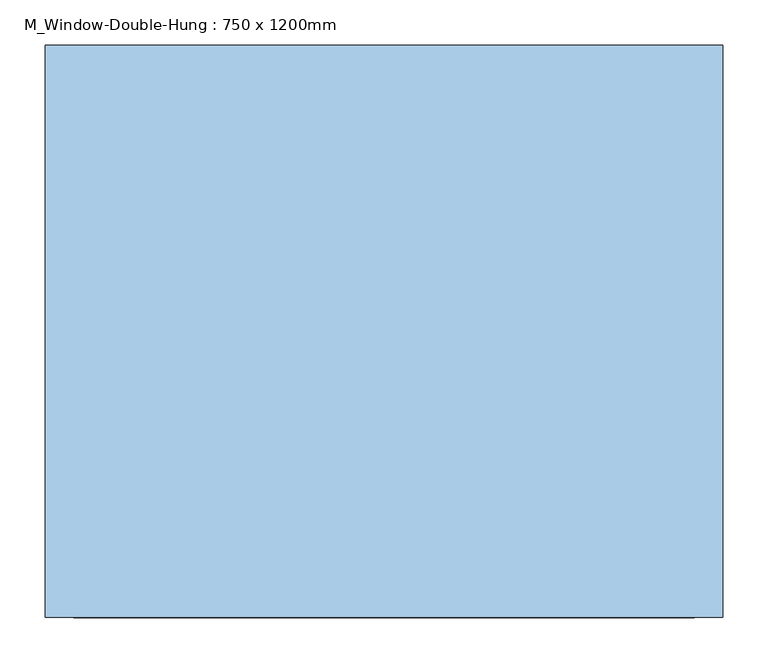
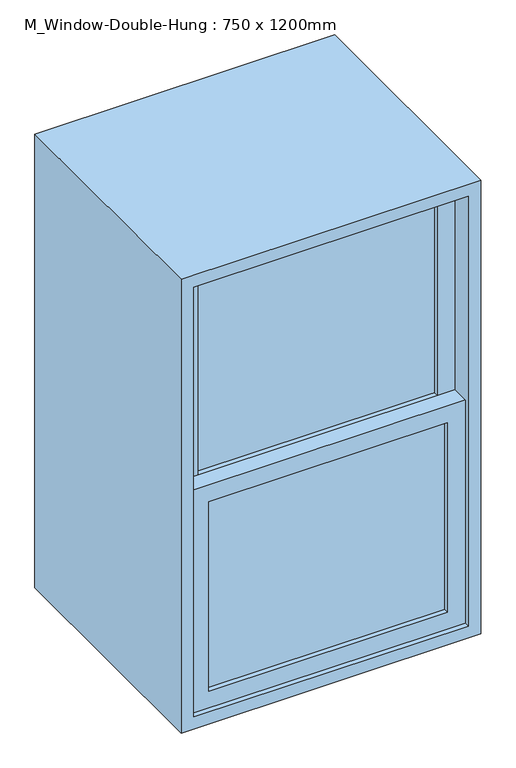
"""IFC4 building model written with IfcOpenShell, lengths in millimetres: window geometry, M_Window-Double-Hung : 750 x 1200mm."""

from ifc_helpers import new_model, si_unit, frame, origin, place, context, project, spatial, polyline, outline, extrude, source, transform, mapped, element, save


def m_window_double_hung_750_x_1200mm_e21ea802(model_context):
    return source(origin(), model_context, "Body", "SweptSolid", [
        extrude(outline(polyline([(298.8, -469.85), (298.8, -476.2), (-298.8, -476.2), (-298.8, -469.85), (298.8, -469.85)])), frame((0.0, 0.0, 990.6), z_axis=(0.0, 0.0, 1.0), x_axis=(1.0, 0.0, 0.0)), (0.0, 0.0, 1.0), 501.575),
        extrude(outline(polyline([(-298.8, -482.55), (298.8, -482.55), (298.8, -488.9), (-298.8, -488.9), (-298.8, -482.55)])), frame((0.0, 0.0, 990.6), z_axis=(0.0, 0.0, 1.0), x_axis=(1.0, 0.0, 0.0)), (0.0, 0.0, 1.0), 501.575),
        extrude(outline(polyline([(298.8, -425.4), (298.8, -431.75), (-298.8, -431.75), (-298.8, -425.4), (298.8, -425.4)])), frame((0.0, 0.0, 1536.625), z_axis=(0.0, 0.0, 1.0), x_axis=(1.0, 0.0, 0.0)), (0.0, 0.0, 1.0), 501.575),
        extrude(outline(polyline([(-298.8, -438.1), (298.8, -438.1), (298.8, -444.45), (-298.8, -444.45), (-298.8, -438.1)])), frame((0.0, 0.0, 1536.625), z_axis=(0.0, 0.0, 1.0), x_axis=(1.0, 0.0, 0.0)), (0.0, 0.0, 1.0), 501.575),
        extrude(outline(polyline([(1536.625, -343.25), (946.15, -343.25), (946.15, 343.25), (1536.625, 343.25), (1536.625, -343.25)]), holes=[polyline([(1492.175, 298.8), (990.6, 298.8), (990.6, -298.8), (1492.175, -298.8), (1492.175, 298.8)])]), frame((0.0, -501.6, 0.0), z_axis=(0.0, 1.0, 0.0), x_axis=(0.0, 0.0, 1.0)), (0.0, 0.0, 1.0), 44.45),
        extrude(outline(polyline([(2082.65, -343.25), (1492.175, -343.25), (1492.175, 343.25), (2082.65, 343.25), (2082.65, -343.25)]), holes=[polyline([(2038.2, 298.8), (1536.625, 298.8), (1536.625, -298.8), (2038.2, -298.8), (2038.2, 298.8)])]), frame((0.0, -457.15, 0.0), z_axis=(0.0, 1.0, 0.0), x_axis=(0.0, 0.0, 1.0)), (0.0, 0.0, 1.0), 44.45),
        extrude(outline(polyline([(2114.4, -375.0), (914.4, -375.0), (914.4, 375.0), (2114.4, 375.0), (2114.4, -375.0)]), holes=[polyline([(2082.65, 343.25), (946.15, 343.25), (946.15, -343.25), (2082.65, -343.25), (2082.65, 343.25)])]), frame((0.0, -514.3, 0.0), z_axis=(0.0, 1.0, 0.0), x_axis=(0.0, 0.0, 1.0)), (0.0, 0.0, 1.0), 633.35),
    ])


if __name__ == "__main__":
    model = new_model("IFC4")
    model_context = context("Model", 3, world=origin())
    ifc_project = project(units=[si_unit("LENGTHUNIT", "METRE", prefix="MILLI")], contexts=[model_context])
    site = spatial("IfcSite", under=ifc_project)
    building = spatial("IfcBuilding", under=site)
    placement = place(None, origin())
    m_window_double_hung_750_x_1200mm_shape = m_window_double_hung_750_x_1200mm_e21ea802(model_context)
    element("IfcWindow", 1, ObjectType="M_Window-Double-Hung : 750 x 1200mm", at=placement, inside=building, context=model_context, shape_type="MappedRepresentation", body=[
        mapped(m_window_double_hung_750_x_1200mm_shape, transform((0.0, 0.0, 0.0), x_axis=(1.0, 0.0, 0.0), y_axis=(0.0, 1.0, 0.0), z_axis=(0.0, 0.0, 1.0))),
    ])
    save(model, "model.ifc")

# Revit data of these elements
# Type "M_Window-Double-Hung : 750 x 1200mm"
#   Type Mark = "22"
#   Fire Rating = "0.5h"
#   Construction Type Id = "DG-DR"
#   Assembly Code = "B2020100"
#   Analytic Construction = "Double glazing - domestic"
#   Wall Thickness [instance default] = 150 mm
#   Window Inset [instance default] = 0 mm
#   Visual Light Transmittance = 0.81
#   Thermal Resistance (R) = 0.319569 (m²·K)/W
#   Solar Heat Gain Coefficient = 0.76
#   Muntin Width = 597.6 mm
#   Muntin Height = 501.575 mm
#   Interior Wall Closure [instance default] = 35.7 mm
#   Rough Width = 765 mm
#   Rough Height = 1215 mm
#   Frame Extension [instance default] = 31.75 mm
#   Exterior Wall Closure [instance default] = 12.7 mm
#   Extension Jamb [instance default] = 35.7 mm
#   Heat Transfer Coefficient (U) = 3.12929 W/(m²·K)
#   Height = 1200 mm
#   Width = 750 mm
#   Define Thermal Properties by = 1
#   Top Muntin Visibility = yes
#   Indicator Visibility [instance default] = yes
#   Extension Jamb Visibility [instance default] = yes
#   Interior Trim Visibility [instance default] = yes
#   Exterior Trim Visibility [instance default] = yes
#   Define Thermal Properties by = 1
#   Bottom Muntin Visibility = yes
#   Muntin Pattern = M_Muntin Pattern_2x2 : M_Muntin Pattern_2x2
#   Interior Trim Material = Wood - Stained
#   Interior Trim = M_Trim-Window-Interior-Flat : Picture Frame
#   Exterior Trim Material = Clad - White
#   Exterior Trim = M_Trim-Window-Exterior-Flat : with Sill
#   Glass Panel Material = Glass
#   Exterior Frame Material = Clad - White
#   Interior Frame Material = Wood - Stained
#   Wall Closure = (empty or 0)
# Element 1 (IfcWindow, "M_Window-Double-Hung : 750 x 1200mm")
#   Wall Thickness = 200 mm
#   Window Inset = 500 mm
#   Frame Extension = 531.75 mm
#   Extension Jamb = 25.4 mm
#   Extension Jamb Visibility = no
#   Materials on its faces: "Wood - Stained", "Glass", "Clad - White"
# Materials
#   "Wood - Stained": class "Wood", colour RGB 224 178 126, transparency 0, Cost = 0
#   "Clad - White": class "Wood", colour RGB 242 242 238, transparency 0, Cost = 0
#   "Glass": class "Glass", colour RGB 0 128 192, transparency 0.9, Description = "Soda Lime Glass", Cost = 0
